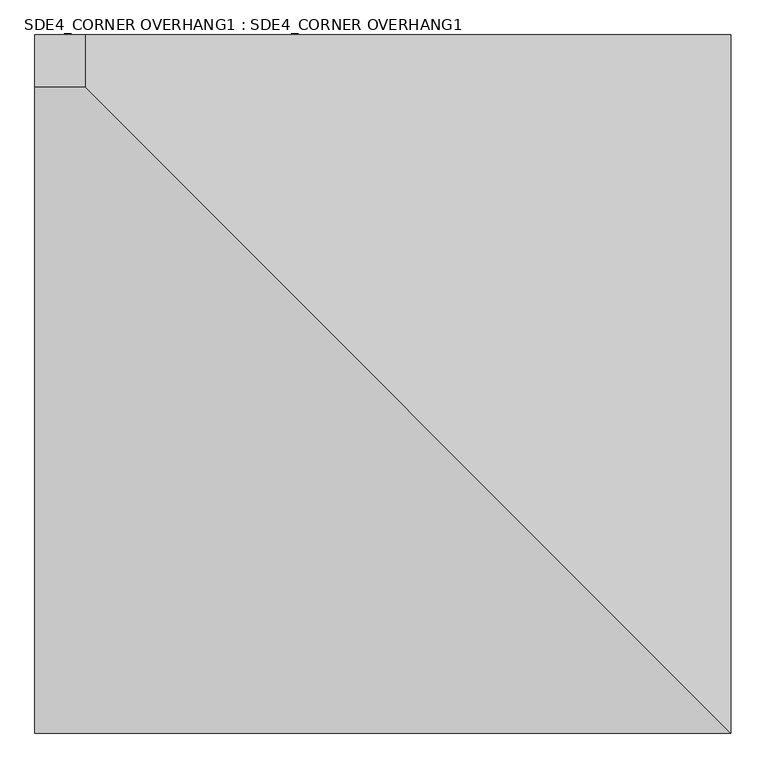
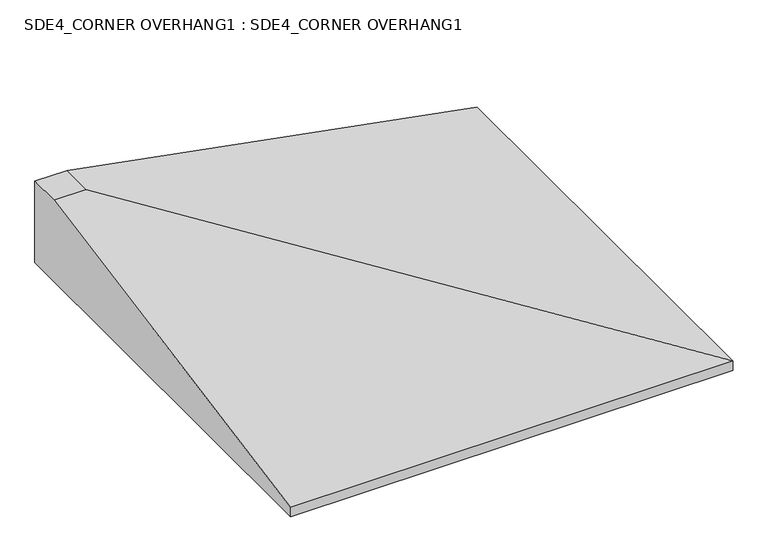
"""IFC4 building model written with IfcOpenShell, lengths in millimetres: proxy geometry, SDE4_CORNER OVERHANG1 : SDE4_CORNER OVERHANG1."""

from ifc_helpers import new_model, si_unit, origin, place, context, project, spatial, faceted_brep, source, transform, mapped, element, save


def sde4_corner_overhang1_sde4_corner_overhang1_ad86b5f8(model_context):
    return source(origin(), model_context, "Body", "Brep", [
        faceted_brep([(73500.4826132, -1544.7500001, 142520.0), (75295.9768176, -1544.7500001, 142520.0), (75295.9768176, -1544.7500001, 142560.0), (73500.4826132, -1544.7500001, 142560.0), (73630.9768176, 255.2499999, 142870.0), (75295.9768176, 255.2499999, 142560.0), (75295.9768176, 255.2499999, 142520.0), (73500.4826132, 255.2499999, 142520.0), (73500.4826132, 255.2499999, 142870.0), (73500.4826132, 120.2499999, 142870.0), (73630.9768176, 120.2499999, 142870.0)], [[[0, 1, 2, 3]], [[4, 5, 6, 7, 8]], [[8, 7, 0, 3, 9]], [[1, 0, 7, 6]], [[2, 1, 6, 5]], [[5, 4, 10, 2]], [[3, 2, 10, 9]], [[4, 8, 9, 10]]]),
    ])


if __name__ == "__main__":
    model = new_model("IFC4")
    model_context = context("Model", 3, world=origin())
    ifc_project = project(units=[si_unit("LENGTHUNIT", "METRE", prefix="MILLI")], contexts=[model_context])
    site = spatial("IfcSite", under=ifc_project)
    building = spatial("IfcBuilding", under=site)
    placement = place(None, origin())
    sde4_corner_overhang1_sde4_corner_overhang1_shape = sde4_corner_overhang1_sde4_corner_overhang1_ad86b5f8(model_context)
    element("IfcBuildingElementProxy", 1, Name="SDE4_CORNER OVERHANG1 : SDE4_CORNER OVERHANG1", ObjectType="SDE4_CORNER OVERHANG1 : SDE4_CORNER OVERHANG1", at=placement, inside=building, context=model_context, shape_type="MappedRepresentation", body=[
        mapped(sde4_corner_overhang1_sde4_corner_overhang1_shape, transform((0.0, 0.0, 0.0), x_axis=(1.0, 0.0, 0.0), y_axis=(0.0, 1.0, 0.0), z_axis=(0.0, 0.0, 1.0))),
    ])
    save(model, "model.ifc")
